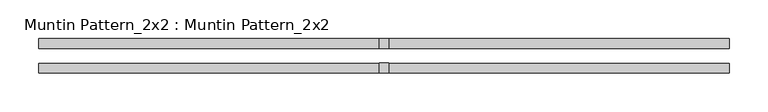
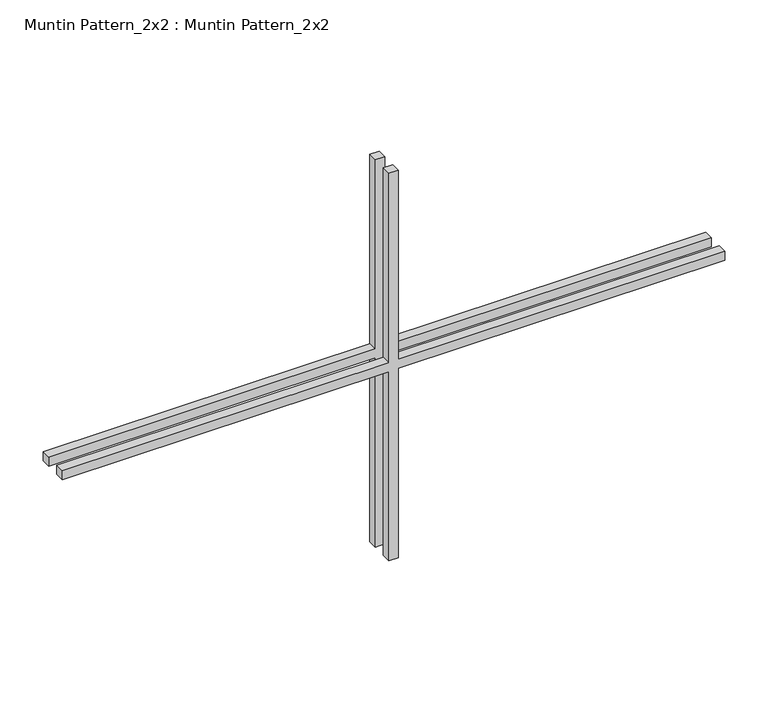
"""IFC4 building model written with IfcOpenShell, lengths in millimetres: proxy geometry, Muntin Pattern_2x2 : Muntin Pattern_2x2."""

from ifc_helpers import new_model, si_unit, frame, origin, place, context, project, spatial, polyline, outline, extrude, source, transform, mapped, element, save


def muntin_pattern_2x2_muntin_pattern_2x2_841f7581(model_context):
    return source(origin(), model_context, "Body", "SweptSolid", [
        extrude(outline(polyline([(280.9875, -6.35), (280.9875, -444.5), (268.2875, -444.5), (268.2875, -6.35), (0.0, -6.35), (0.0, 6.35), (268.2875, 6.35), (268.2875, 444.5), (280.9875, 444.5), (280.9875, 6.35), (549.275, 6.35), (549.275, -6.35), (280.9875, -6.35)])), frame((0.0, 9.525, 0.0), z_axis=(0.0, 1.0, 0.0), x_axis=(0.0, 0.0, 1.0)), (0.0, 0.0, 1.0), 12.7),
        extrude(outline(polyline([(280.9875, -6.35), (280.9875, -444.5), (268.2875, -444.5), (268.2875, -6.35), (0.0, -6.35), (0.0, 6.35), (268.2875, 6.35), (268.2875, 444.5), (280.9875, 444.5), (280.9875, 6.35), (549.275, 6.35), (549.275, -6.35), (280.9875, -6.35)])), frame((0.0, -22.225, 0.0), z_axis=(0.0, 1.0, 0.0), x_axis=(0.0, 0.0, 1.0)), (0.0, 0.0, 1.0), 12.7),
    ])


if __name__ == "__main__":
    model = new_model("IFC4")
    model_context = context("Model", 3, world=origin())
    ifc_project = project(units=[si_unit("LENGTHUNIT", "METRE", prefix="MILLI")], contexts=[model_context])
    site = spatial("IfcSite", under=ifc_project)
    building = spatial("IfcBuilding", under=site)
    placement = place(None, origin())
    muntin_pattern_2x2_muntin_pattern_2x2_shape = muntin_pattern_2x2_muntin_pattern_2x2_841f7581(model_context)
    element("IfcBuildingElementProxy", 1, Name="Muntin Pattern_2x2 : Muntin Pattern_2x2", ObjectType="Muntin Pattern_2x2 : Muntin Pattern_2x2", at=placement, inside=building, context=model_context, shape_type="MappedRepresentation", body=[
        mapped(muntin_pattern_2x2_muntin_pattern_2x2_shape, transform((0.0, 0.0, 0.0), x_axis=(1.0, 0.0, 0.0), y_axis=(0.0, 1.0, 0.0), z_axis=(0.0, 0.0, 1.0))),
    ])
    save(model, "model.ifc")

# Revit data of these elements
# Type "Muntin Pattern_2x2 : Muntin Pattern_2x2"
#   Width [instance default] = 4' - 0"
#   Thickness = 0' - 0 1/2"
#   Height [instance default] = 4' - 0"
#   Distance = 0' - 0 3/4"
#   Interior Material [instance default] = none
#   Exterior Material [instance default] = none
# Element 1 (IfcBuildingElementProxy, "Muntin Pattern_2x2 : Muntin Pattern_2x2")
#   Width = 2' - 11"
#   Height = 1' - 9 5/8"
#   Interior Material = Wood - Stained
#   Exterior Material = Clad - White
#   Materials on its faces: "Clad - White", "Wood - Stained"
# Materials
#   "Clad - White": class "Wood", colour RGB 242 242 238, transparency 0, Cost = 0
#   "Wood - Stained": class "Wood", colour RGB 224 178 126, transparency 0, Cost = 0
